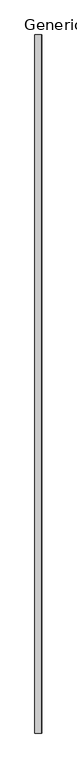
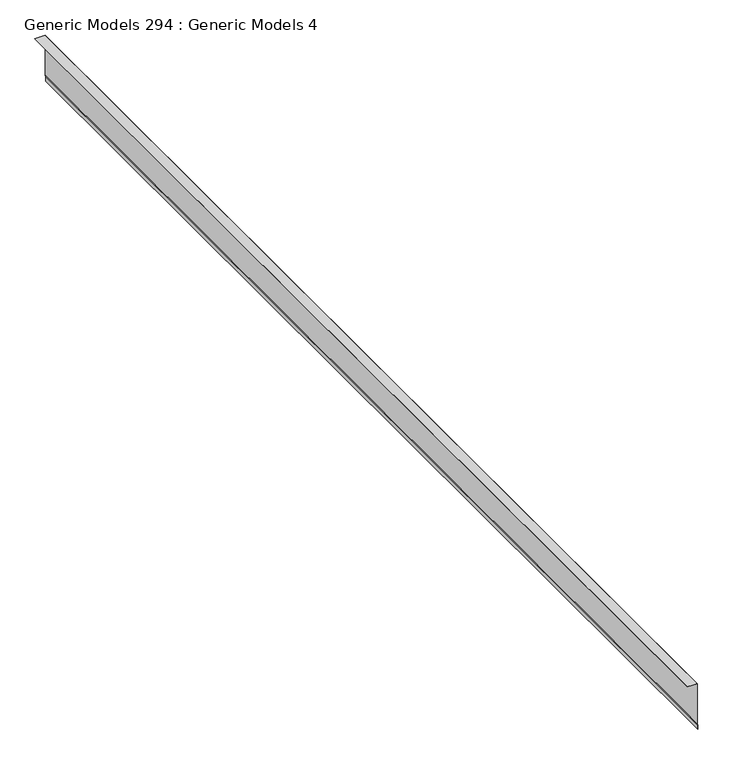
"""IFC4 building model written with IfcOpenShell, lengths in millimetres: proxy geometry, Generic Models 294 : Generic Models 4."""

from ifc_helpers import new_model, si_unit, frame, origin, place, context, project, spatial, polyline, outline, extrude, source, transform, mapped, element, save


def generic_models_294_generic_models_4_5ee858b6(model_context):
    return source(origin(), model_context, "Body", "SweptSolid", [
        extrude(outline(polyline([(124892.7420872, 4943.1131476), (124477.2202016, 4943.1131476), (124456.3128095, 4950.722816), (124413.7059626, 4950.722816), (124413.7059626, 4951.516566), (124456.452769, 4951.516566), (124477.3601612, 4943.9068976), (124893.5358372, 4943.9068976), (124893.5358372, 4843.7488769), (124892.7420872, 4843.7488769), (124892.7420872, 4943.1131476)])), frame((0.0, -2626.9952162, 0.0), z_axis=(0.0, 1.0, 0.0), x_axis=(0.0, 0.0, 1.0)), (0.0, 0.0, 1.0), 11105.6544692),
    ])


if __name__ == "__main__":
    model = new_model("IFC4")
    model_context = context("Model", 3, world=origin())
    ifc_project = project(units=[si_unit("LENGTHUNIT", "METRE", prefix="MILLI")], contexts=[model_context])
    site = spatial("IfcSite", under=ifc_project)
    building = spatial("IfcBuilding", under=site)
    placement = place(None, origin())
    generic_models_294_generic_models_4_shape = generic_models_294_generic_models_4_5ee858b6(model_context)
    element("IfcBuildingElementProxy", 1, Name="Generic Models 294 : Generic Models 4", ObjectType="Generic Models 294 : Generic Models 4", at=placement, inside=building, context=model_context, shape_type="MappedRepresentation", body=[
        mapped(generic_models_294_generic_models_4_shape, transform((0.0, 0.0, 0.0), x_axis=(1.0, 0.0, 0.0), y_axis=(0.0, 1.0, 0.0), z_axis=(0.0, 0.0, 1.0))),
    ])
    save(model, "model.ifc")

# Revit data of these elements
# Element 1 (IfcBuildingElementProxy, "Generic Models 294 : Generic Models 4")
#   Materials on its faces: "_(2) LAYERS NO. 30 ASTM D226 ASPHALT SATURATED ORGANIC FELT"
# Materials
#   "_(2) LAYERS NO. 30 ASTM D226 ASPHALT SATURATED ORGANIC FELT": class "Generic", colour RGB 67 154 161, transparency 0, Cost = 0
